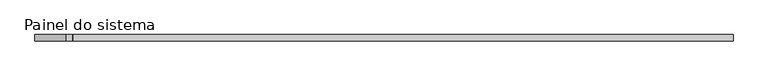
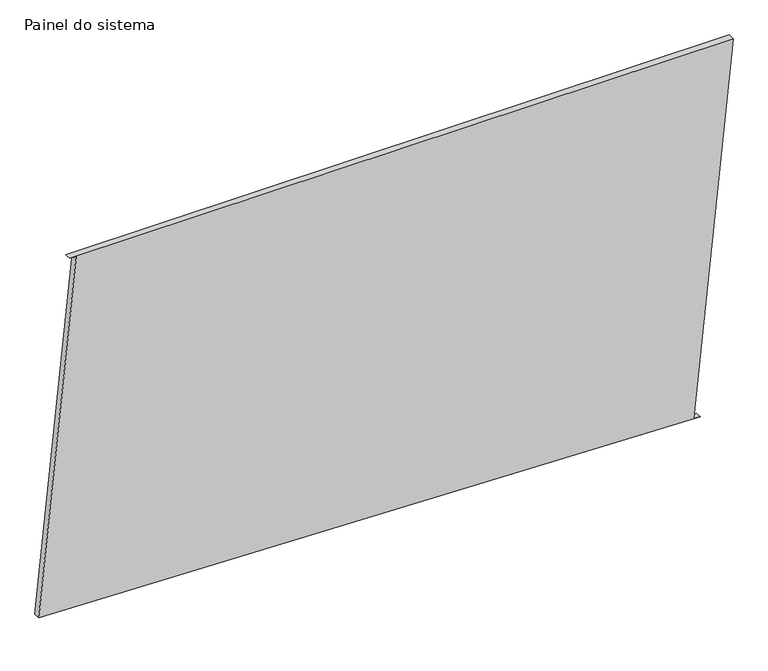
"""IFC4 building model written with IfcOpenShell, lengths in millimetres: plate geometry, Painel do sistema : Envidraçado."""

from ifc_helpers import new_model, si_unit, frame, origin, place, context, project, spatial, polyline, outline, extrude, source, transform, mapped, element, save


def painel_do_sistema_70a71ee5(model_context):
    return source(origin(), model_context, "Body", "SweptSolid", [
        extrude(outline(polyline([(0.0, 1213.006923), (2.5300763, 1188.1352782), (1498.5622027, 1340.3196414), (1498.5622027, -1220.4568583), (1496.0321264, -1195.5852135), (73.2357927, -1340.3196414), (0.0, 1213.006923)])), frame((0.0, 24.5, 0.0), z_axis=(0.0, 1.0, 0.0), x_axis=(0.0, 0.0, 1.0)), (0.0, 0.0, 1.0), 25.0),
    ])


if __name__ == "__main__":
    model = new_model("IFC4")
    model_context = context("Model", 3, world=origin())
    ifc_project = project(units=[si_unit("LENGTHUNIT", "METRE", prefix="MILLI")], contexts=[model_context])
    site = spatial("IfcSite", under=ifc_project)
    building = spatial("IfcBuilding", under=site)
    placement = place(None, origin())
    painel_do_sistema_shape = painel_do_sistema_70a71ee5(model_context)
    element("IfcPlate", 1, ObjectType="Painel do sistema : Envidraçado", at=placement, inside=building, context=model_context, shape_type="MappedRepresentation", body=[
        mapped(painel_do_sistema_shape, transform((0.0, 0.0, 0.0), x_axis=(1.0, 0.0, 0.0), y_axis=(0.0, 1.0, 0.0), z_axis=(0.0, 0.0, 1.0))),
    ])
    save(model, "model.ifc")

# Revit data of these elements
# Type "Painel do sistema : Envidraçado"
#   Construction Type Id = "GSP4R"
#   Analytic Construction = "Vidraça única Pilkington 1/8 pol"
#   Visual Light Transmittance = 0.9
#   Solar Heat Gain Coefficient = 0.86
#   Heat Transfer Coefficient (U) = 6.7069 W/(m²·K)
# Element 1 (IfcPlate, "Painel do sistema : Envidraçado")
#   Materials on its faces: "Vidro"
# Materials
#   "Vidro": class "Vidro", colour RGB 0 128 192, transparency 0.9, Description = "Vidro de sílica", Cost = 0
